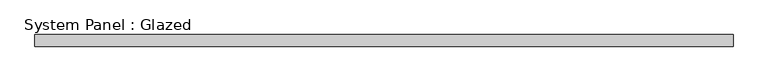
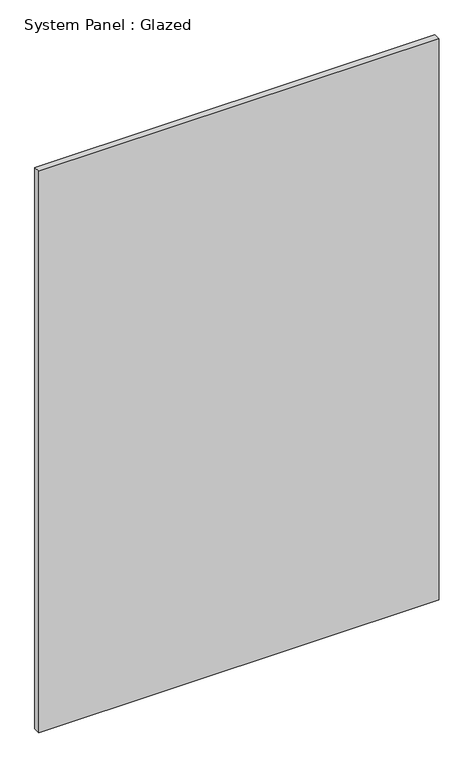
"""IFC4 building model written with IfcOpenShell, lengths in millimetres: plate geometry, System Panel : Glazed."""

from ifc_helpers import new_model, si_unit, origin, origin_with_axes, place, context, project, spatial, polyline, outline, extrude, source, transform, mapped, element, save


def system_panel_glazed_8f795733(model_context):
    return source(origin(), model_context, "Body", "SweptSolid", [
        extrude(outline(polyline([(725.0514967, -49.5), (-725.0514967, -49.5), (-725.0514967, -24.5), (725.0514967, -24.5), (725.0514967, -49.5)])), origin_with_axes(), (0.0, 0.0, 1.0), 2150.0),
    ])


if __name__ == "__main__":
    model = new_model("IFC4")
    model_context = context("Model", 3, world=origin())
    ifc_project = project(units=[si_unit("LENGTHUNIT", "METRE", prefix="MILLI")], contexts=[model_context])
    site = spatial("IfcSite", under=ifc_project)
    building = spatial("IfcBuilding", under=site)
    placement = place(None, origin())
    system_panel_glazed_shape = system_panel_glazed_8f795733(model_context)
    element("IfcPlate", 1, ObjectType="System Panel : Glazed", at=placement, inside=building, context=model_context, shape_type="MappedRepresentation", body=[
        mapped(system_panel_glazed_shape, transform((0.0, 0.0, 0.0), x_axis=(1.0, 0.0, 0.0), y_axis=(0.0, 1.0, 0.0), z_axis=(0.0, 0.0, 1.0))),
    ])
    save(model, "model.ifc")

# Revit data of these elements
# Type "System Panel : Glazed"
#   Keynote = "H11"
#   Construction Type Id = "GSP4R"
#   Analytic Construction = "1/8 in Pilkington single glazing"
#   Visual Light Transmittance = 0.9
#   Solar Heat Gain Coefficient = 0.86
#   Heat Transfer Coefficient (U) = 6.7069 W/(m²·K)
# Element 1 (IfcPlate, "System Panel : Glazed")
#   Materials on its faces: "Glass"
# Materials
#   "Glass": class "Glass", colour RGB 0 128 192, transparency 0.9, Description = "Soda Lime Glass", Cost = 0
